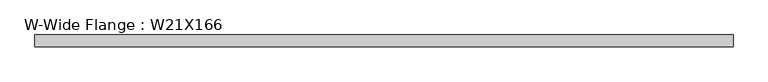
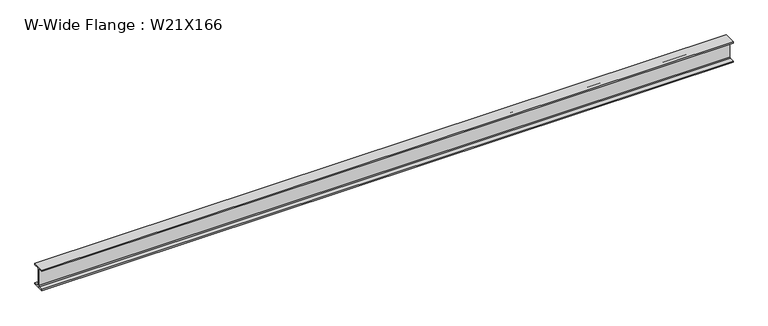
"""IFC4 building model written with IfcOpenShell, lengths in millimetres: beam geometry, W-Wide Flange : W21X166."""

from ifc_helpers import new_model, si_unit, point, frame, frame_2d, origin, place, context, project, spatial, polyline, circle_curve, trimmed, segment, composite_curve, outline, extrude, source, transform, mapped, element, save


def w_wide_flange_w21x166_70861c47(model_context):
    return source(origin(), model_context, "Body", "SweptSolid", [
        extrude(outline(composite_curve([segment(polyline([(157.48, -251.206), (157.48, -285.75), (-157.48, -285.75), (-157.48, -251.206), (-32.131, -251.206)]), True, "CONTINUOUS"), segment(trimmed(circle_curve(frame_2d((-32.131, -228.6)), 22.606), [point((-32.131, -251.206))], [point((-9.525, -228.6))], True, "CARTESIAN"), True, "CONTINUOUS"), segment(polyline([(-9.525, -228.6), (-9.525, 228.6)]), True, "CONTINUOUS"), segment(trimmed(circle_curve(frame_2d((-32.131, 228.6)), 22.606), [point((-9.525, 228.6))], [point((-32.131, 251.206))], True, "CARTESIAN"), True, "CONTINUOUS"), segment(polyline([(-32.131, 251.206), (-157.48, 251.206), (-157.48, 285.75), (157.48, 285.75), (157.48, 251.206), (32.131, 251.206)]), True, "CONTINUOUS"), segment(trimmed(circle_curve(frame_2d((32.131, 228.6)), 22.606), [point((32.131, 251.206))], [point((9.525, 228.6))], True, "CARTESIAN"), True, "CONTINUOUS"), segment(polyline([(9.525, 228.6), (9.525, -228.6)]), True, "CONTINUOUS"), segment(trimmed(circle_curve(frame_2d((32.131, -228.6)), 22.606), [point((9.525, -228.6))], [point((32.131, -251.206))], True, "CARTESIAN"), True, "CONTINUOUS"), segment(polyline([(32.131, -251.206), (157.48, -251.206)]), True, "CONTINUOUS")], self_intersect=False)), frame((-9109.5045465, 0.0, 0.0), z_axis=(1.0, 0.0, 0.0), x_axis=(0.0, 1.0, 0.0)), (0.0, 0.0, 1.0), 18197.9516916),
    ])


if __name__ == "__main__":
    model = new_model("IFC4")
    model_context = context("Model", 3, world=origin())
    ifc_project = project(units=[si_unit("LENGTHUNIT", "METRE", prefix="MILLI")], contexts=[model_context])
    site = spatial("IfcSite", under=ifc_project)
    building = spatial("IfcBuilding", under=site)
    placement = place(None, origin())
    w_wide_flange_w21x166_shape = w_wide_flange_w21x166_70861c47(model_context)
    element("IfcBeam", 1, ObjectType="W-Wide Flange : W21X166", at=placement, inside=building, context=model_context, shape_type="MappedRepresentation", body=[
        mapped(w_wide_flange_w21x166_shape, transform((0.0, 0.0, 0.0), x_axis=(1.0, 0.0, 0.0), y_axis=(0.0, 1.0, 0.0), z_axis=(0.0, 0.0, 1.0))),
    ])
    save(model, "model.ifc")

# Revit data of these elements
# Type "W-Wide Flange : W21X166"
#   Assembly Code = "B10"
#   W = 166
#   Length [instance default] = 5' - 0"
#   bf = 1' - 0.4"
#   d = 1' - 10 1/2"
#   k = 0' - 2 1/4"
#   k2 = 0' - 0.89"
#   tf = 0' - 1.36"
#   tw = 0' - 0 3/4"
#   A = 0.338889 SF
#   Structural Material [instance default] = Steel ASTM A992
# Element 1 (IfcBeam, "W-Wide Flange : W21X166")
#   Structural Material = Steel
#   Materials on its faces: "Steel"
# Materials
#   "Steel ASTM A992": class "Metal", colour RGB 199 199 199, transparency 0, Description = "Structural steel 50ksi", Cost = 0
#   "Steel": class "Metal", colour RGB 118 118 114, transparency 0, Description = "Steel, mill finish", Cost = 0
